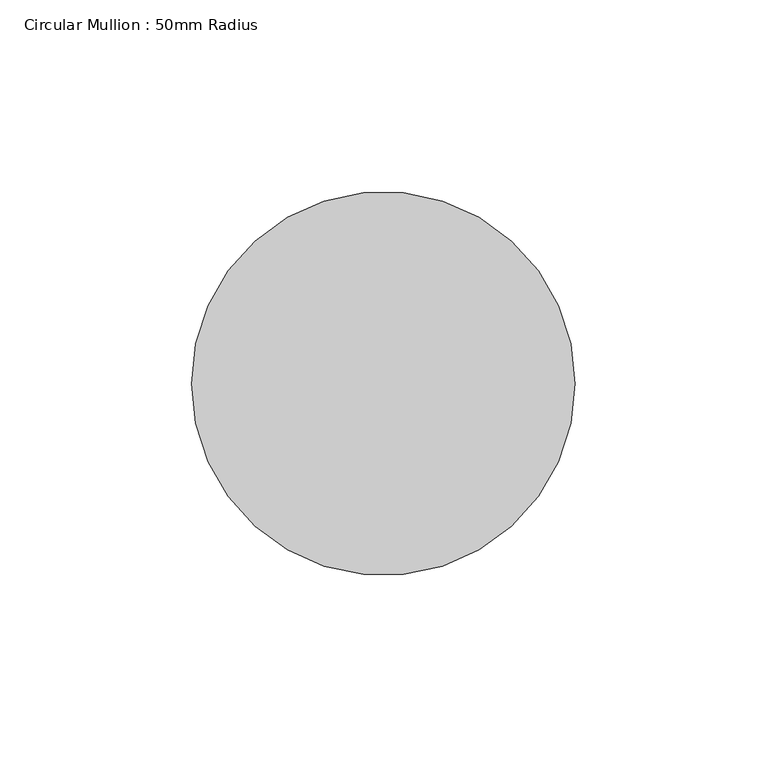
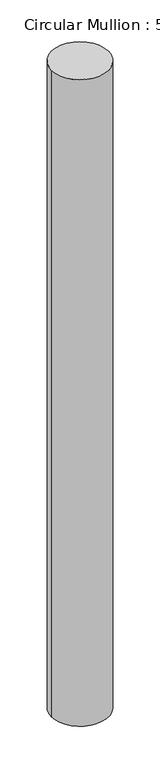
"""IFC4 building model written with IfcOpenShell, lengths in millimetres: member geometry, Circular Mullion : 50mm Radius."""

from ifc_helpers import new_model, si_unit, point, frame, origin, origin_2d, place, context, project, spatial, circle_curve, trimmed, segment, composite_curve, outline, extrude, source, transform, mapped, element, save


def circular_mullion_50mm_radius_80557375(model_context):
    return source(origin(), model_context, "Body", "SweptSolid", [
        extrude(outline(composite_curve([segment(trimmed(circle_curve(origin_2d(), 50.0), [point((50.0, 0.0))], [point((-50.0, 0.0))], False, "CARTESIAN"), True, "CONTINUOUS"), segment(trimmed(circle_curve(origin_2d(), 50.0), [point((-50.0, 0.0))], [point((50.0, 0.0))], False, "CARTESIAN"), True, "CONTINUOUS")], self_intersect=False)), frame((0.0, 0.0, -1196.6863777), z_axis=(0.0, 0.0, 1.0), x_axis=(1.0, 0.0, 0.0)), (0.0, 0.0, 1.0), 1196.6863777),
    ])


if __name__ == "__main__":
    model = new_model("IFC4")
    model_context = context("Model", 3, world=origin())
    ifc_project = project(units=[si_unit("LENGTHUNIT", "METRE", prefix="MILLI")], contexts=[model_context])
    site = spatial("IfcSite", under=ifc_project)
    building = spatial("IfcBuilding", under=site)
    placement = place(None, origin())
    circular_mullion_50mm_radius_shape = circular_mullion_50mm_radius_80557375(model_context)
    element("IfcMember", 1, ObjectType="Circular Mullion : 50mm Radius", at=placement, inside=building, context=model_context, shape_type="MappedRepresentation", body=[
        mapped(circular_mullion_50mm_radius_shape, transform((0.0, 0.0, 0.0), x_axis=(1.0, 0.0, 0.0), y_axis=(0.0, 1.0, 0.0), z_axis=(0.0, 0.0, 1.0))),
    ])
    save(model, "model.ifc")

# Revit data of these elements
# Type "Circular Mullion : 50mm Radius"
#   built-in parameter 1007350 = 0.164042 (stored number, unit not read)
# Element 1 (IfcMember, "Circular Mullion : 50mm Radius")
#   Materials on its faces: "Aluminium"
# Materials
#   "Aluminium": class "Metal", colour RGB 247 247 247, transparency 0, Description = "Aluminium 6061", Cost = 0
